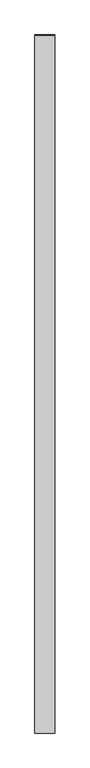
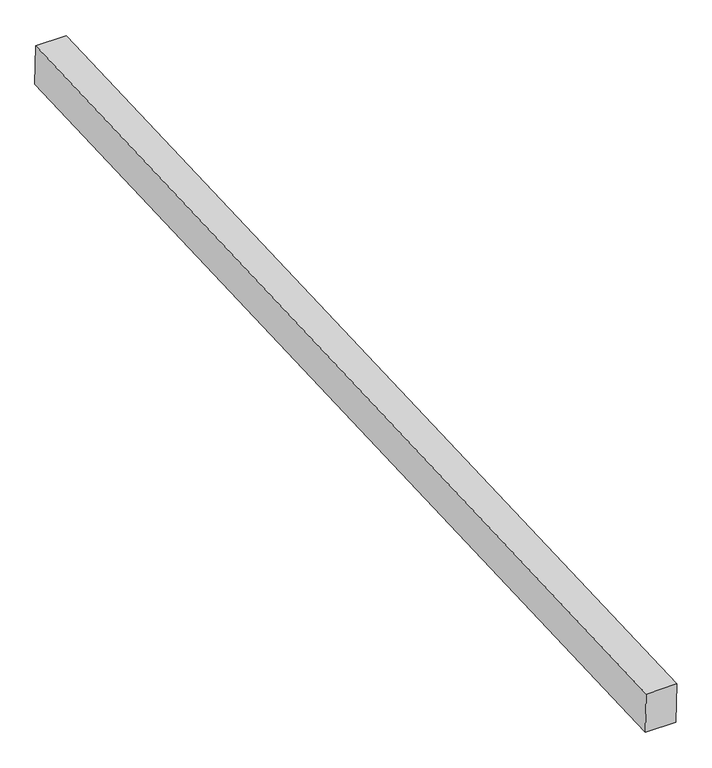
"""IFC4 building model written with IfcOpenShell, lengths in millimetres: proxy geometry, Generic Models 7:Generic Models 1:8:Generic Models 1:8 : Generic Models 7:Generic Models 1:337419:42 : Generic Models 7:Generic Models 1:8:Generic Models 1:8 : Generic Models 7:Generic Models 1:337419:315935."""

from ifc_helpers import new_model, si_unit, frame, origin, place, context, project, spatial, polyline, outline, extrude, source, transform, mapped, element, save


def generic_models_47fd37d5(model_context):
    return source(origin(), model_context, "Body", "SweptSolid", [
        extrude(outline(polyline([(-581229.2495411, 3818.908703), (-576356.3266468, 4021.9471569), (-576348.7597251, 3831.5971524), (-581221.3189223, 3628.5738526), (-581229.2495411, 3818.908703)])), frame((662295.8617239, 0.0, 0.0), z_axis=(1.0, 0.0, 0.0), x_axis=(0.0, 1.0, 0.0)), (0.0, 0.0, 1.0), 139.7),
    ])


if __name__ == "__main__":
    model = new_model("IFC4")
    model_context = context("Model", 3, world=origin())
    ifc_project = project(units=[si_unit("LENGTHUNIT", "METRE", prefix="MILLI")], contexts=[model_context])
    site = spatial("IfcSite", under=ifc_project)
    building = spatial("IfcBuilding", under=site)
    placement = place(None, origin())
    generic_models_shape = generic_models_47fd37d5(model_context)
    element("IfcBuildingElementProxy", 1, Name="Generic Models 7:Generic Models 1:8:Generic Models 1:8 : Generic Models 7:Generic Models 1:337419:42 : Generic Models 7:Generic Models 1:8:Generic Models 1:8 : Generic Models 7:Generic Models 1:337419:315935", ObjectType="Generic Models 7:Generic Models 1:8:Generic Models 1:8 : Generic Models 7:Generic Models 1:337419:42 : Generic Models 7:Generic Models 1:8:Generic Models 1:8 : Generic Models 7:Generic Models 1:337419:315935", at=placement, inside=building, context=model_context, shape_type="MappedRepresentation", body=[
        mapped(generic_models_shape, transform((0.0, 0.0, 0.0), x_axis=(1.0, 0.0, 0.0), y_axis=(0.0, 1.0, 0.0), z_axis=(0.0, 0.0, 1.0))),
    ])
    save(model, "model.ifc")

# Revit data of these elements
# Type "Generic Models 7:Generic Models 1:8:Generic Models 1:8 : Generic Models 7:Generic Models 1:337419:42 : Generic Models 7:Generic Models 1:8:Generic Models 1:8 : Generic Models 7:Generic Models 1:337419:315935"
#   NameOverride = "Generic Models 7:Generic Models 1:8:Generic Models 1:8 : Generic Models 7:Generic Models 1:337419:315935"
#   ObjectTypeOverride = "Generic Models 1:8 : Generic Models 7:Generic Models 1:337419"
#   Reference = "Generic Models 1"
#   Tag = "315935"
# Element 1 (IfcBuildingElementProxy, "Generic Models 7:Generic Models 1:8:Generic Models 1:8 : Generic Models 7:Generic Models 1:337419:42 : Generic Models 7:Generic Models 1:8:Generic Models 1:8 : Generic Models 7:Generic Models 1:337419:315935")
#   Materials on its faces: "5 1/2\" X 7 1/2\" EXTERIOR GRADE GLULAM BEAMS"
# Materials
#   "5 1/2\" X 7 1/2\" EXTERIOR GRADE GLULAM BEAMS": class "Wood", colour RGB 183 134 68, transparency 0, Keynote = "M06181300.01", Description = "Pinus Echinata", Cost = 0
